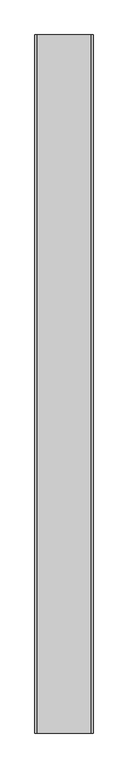
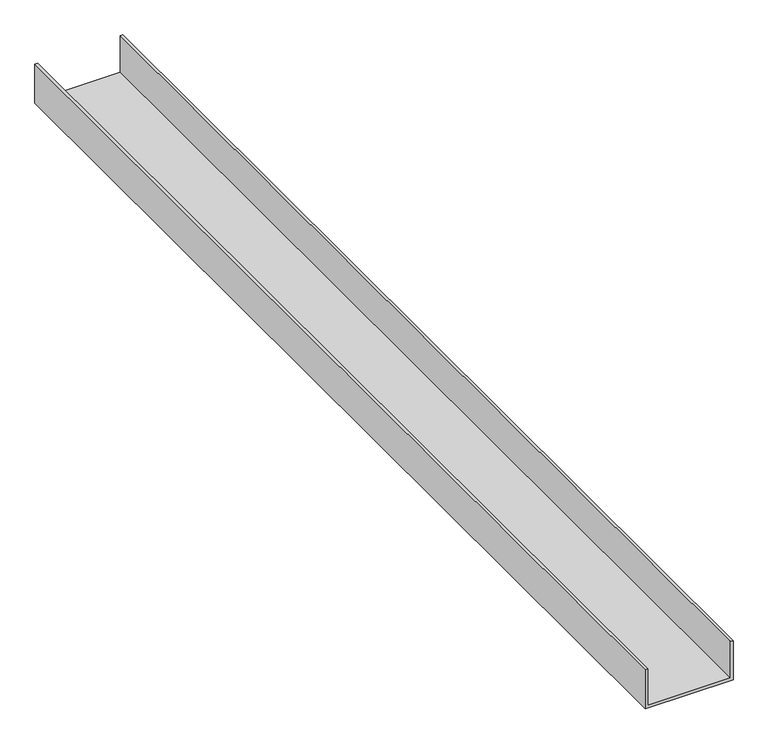
"""IFC4 building model written with IfcOpenShell, lengths in millimetres: proxy geometry, Generic Models 3:Generic Models 1:6:Generic Models 1:6 : Generic Models 3:Generic Models 1:300625:350611:Generic Models 1:6:Generic Models 1:6 : Generic Models 3:Generic Models 1:300625:350611 : Generic Models 3:Generic Models 1:6:Generic Models 1:6 : Generic Models 3:Generic Models 1:300625:350611:3 : Generic Models 3:Generic Models 1:6:Generic Models 1:6 : Generic Models 3:Generic Models 1:300625:350611:Generic Models 1:6:Generic Models 1:6 : Generic Models 3:Generic Models 1:300625:350611 : Generic Models 3:Generic Models 1:6:Generic Models 1:6 : Generic Models 3:Generic Models 1:300625:350611:301824."""

from ifc_helpers import new_model, si_unit, frame, origin, place, context, project, spatial, polyline, outline, extrude, source, transform, mapped, element, save


def generic_models_33e349aa(model_context):
    return source(origin(), model_context, "Body", "SweptSolid", [
        extrude(outline(polyline([(0.0, 560568.8617239), (95.25, 560568.8617239), (95.25, 560562.5117239), (6.35, 560562.5117239), (6.35, 560372.0117239), (95.25, 560372.0117239), (95.25, 560365.6617239), (0.0, 560365.6617239), (0.0, 560568.8617239)])), frame((0.0, -545628.2663841, 0.0), z_axis=(0.0, 1.0, 0.0), x_axis=(0.0, 0.0, 1.0)), (0.0, 0.0, 1.0), 2438.4),
    ])


if __name__ == "__main__":
    model = new_model("IFC4")
    model_context = context("Model", 3, world=origin())
    ifc_project = project(units=[si_unit("LENGTHUNIT", "METRE", prefix="MILLI")], contexts=[model_context])
    site = spatial("IfcSite", under=ifc_project)
    building = spatial("IfcBuilding", under=site)
    placement = place(None, origin())
    generic_models_shape = generic_models_33e349aa(model_context)
    element("IfcBuildingElementProxy", 1, Name="Generic Models 3:Generic Models 1:6:Generic Models 1:6 : Generic Models 3:Generic Models 1:300625:350611:Generic Models 1:6:Generic Models 1:6 : Generic Models 3:Generic Models 1:300625:350611 : Generic Models 3:Generic Models 1:6:Generic Models 1:6 : Generic Models 3:Generic Models 1:300625:350611:3 : Generic Models 3:Generic Models 1:6:Generic Models 1:6 : Generic Models 3:Generic Models 1:300625:350611:Generic Models 1:6:Generic Models 1:6 : Generic Models 3:Generic Models 1:300625:350611 : Generic Models 3:Generic Models 1:6:Generic Models 1:6 : Generic Models 3:Generic Models 1:300625:350611:301824", ObjectType="Generic Models 3:Generic Models 1:6:Generic Models 1:6 : Generic Models 3:Generic Models 1:300625:350611:Generic Models 1:6:Generic Models 1:6 : Generic Models 3:Generic Models 1:300625:350611 : Generic Models 3:Generic Models 1:6:Generic Models 1:6 : Generic Models 3:Generic Models 1:300625:350611:3 : Generic Models 3:Generic Models 1:6:Generic Models 1:6 : Generic Models 3:Generic Models 1:300625:350611:Generic Models 1:6:Generic Models 1:6 : Generic Models 3:Generic Models 1:300625:350611 : Generic Models 3:Generic Models 1:6:Generic Models 1:6 : Generic Models 3:Generic Models 1:300625:350611:301824", at=placement, inside=building, context=model_context, shape_type="MappedRepresentation", body=[
        mapped(generic_models_shape, transform((0.0, 0.0, 0.0), x_axis=(1.0, 0.0, 0.0), y_axis=(0.0, 1.0, 0.0), z_axis=(0.0, 0.0, 1.0))),
    ])
    save(model, "model.ifc")

# Revit data of these elements
# Type "Generic Models 3:Generic Models 1:6:Generic Models 1:6 : Generic Models 3:Generic Models 1:300625:350611:Generic Models 1:6:Generic Models 1:6 : Generic Models 3:Generic Models 1:300625:350611 : Generic Models 3:Generic Models 1:6:Generic Models 1:6 : Generic Models 3:Generic Models 1:300625:350611:3 : Generic Models 3:Generic Models 1:6:Generic Models 1:6 : Generic Models 3:Generic Models 1:300625:350611:Generic Models 1:6:Generic Models 1:6 : Generic Models 3:Generic Models 1:300625:350611 : Generic Models 3:Generic Models 1:6:Generic Models 1:6 : Generic Models 3:Generic Models 1:300625:350611:301824"
#   NameOverride = "Generic Models 3:Generic Models 1:6:Generic Models 1:6 : Generic Models 3:Generic Models 1:300625:350611:Generic Models 1:6:Generic Models 1:6 : Generic Models 3:Generic Models 1:300625:350611 : Generic Models 3:Generic Models 1:6:Generic Models 1:6 : Generic Models 3:Generic Models 1:300625:350611:301824"
#   ObjectTypeOverride = "Generic Models 1:6:Generic Models 1:6 : Generic Models 3:Generic Models 1:300625:350611 : Generic Models 3:Generic Models 1:6:Generic Models 1:6 : Generic Models 3:Generic Models 1:300625:350611"
#   Reference = "Generic Models 1"
#   Tag = "301824"
